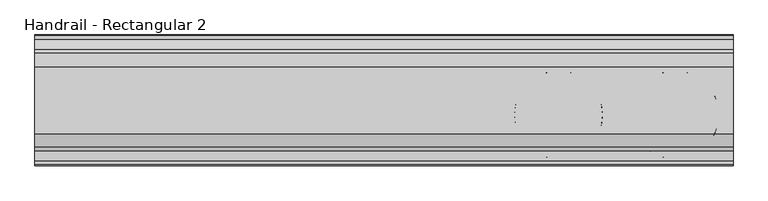
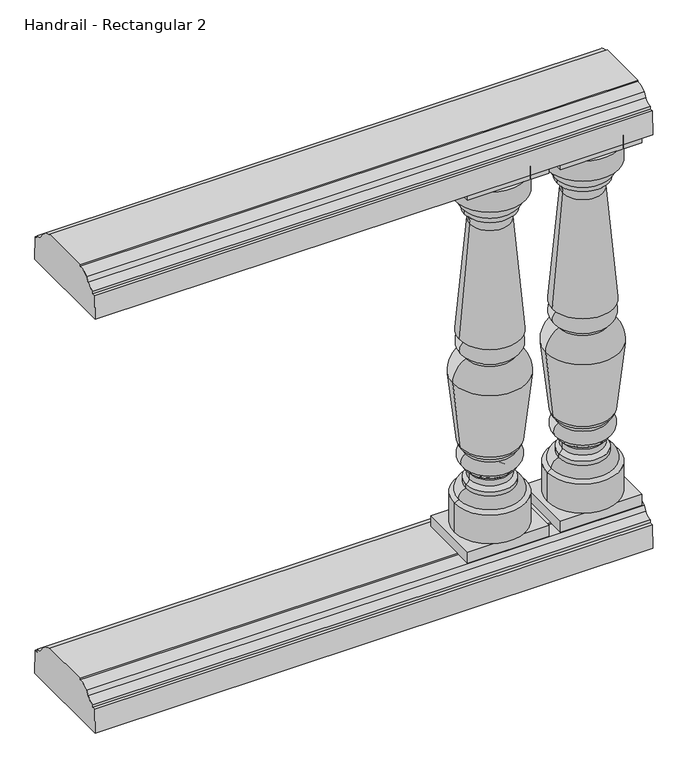
"""IFC4 building model written with IfcOpenShell, lengths in millimetres: railing geometry, Handrail - Rectangular 2."""

from ifc_helpers import new_model, si_unit, point, frame, frame_2d, origin, place, context, project, spatial, polyline, circle_curve, ellipse_curve, trimmed, segment, composite_curve, outline, extrude, source, transform, mapped, element, save
from ifc_brep_helpers import plane_surface, cylinder_surface, revolved_surface, advanced_brep


def handrail_rectangular_2_3b62de76(model_context):
    return source(origin(), model_context, "Body", "SolidModel", [
        extrude(outline(composite_curve([segment(trimmed(circle_curve(frame_2d((-1771.1852268, 1054.89375)), 19.84375), [point((-1771.1852268, 1035.05))], [point((-1754.064785, 1044.8605607))], True, "CARTESIAN"), True, "CONTINUOUS"), segment(polyline([(-1754.064785, 1044.8605607), (-1747.604713, 1054.3201059)]), True, "CONTINUOUS"), segment(trimmed(circle_curve(frame_2d((-1723.5602268, 1027.90625)), 35.71875), [point((-1747.604713, 1054.3201059))], [point((-1723.5602268, 1063.625))], False, "CARTESIAN"), True, "CONTINUOUS"), segment(polyline([(-1723.5602268, 1063.625), (-1723.5602268, 1066.8), (-1607.6727268, 1066.8), (-1607.6727268, 1063.625)]), True, "CONTINUOUS"), segment(trimmed(circle_curve(frame_2d((-1607.6727268, 1027.90625)), 35.71875), [point((-1607.6727268, 1063.625))], [point((-1583.6282406, 1054.3201059))], False, "CARTESIAN"), True, "CONTINUOUS"), segment(polyline([(-1583.6282406, 1054.3201059), (-1577.1681686, 1044.8605607)]), True, "CONTINUOUS"), segment(trimmed(circle_curve(frame_2d((-1560.0477268, 1054.89375)), 19.84375), [point((-1577.1681686, 1044.8605607))], [point((-1560.0477268, 1035.05))], True, "CARTESIAN"), True, "CONTINUOUS"), segment(polyline([(-1560.0477268, 1035.05), (-1560.0477268, 1028.7), (-1552.9039768, 1028.7), (-1551.3164768, 974.725), (-1779.9164768, 974.725), (-1778.3289768, 1028.7), (-1771.1852268, 1028.7), (-1771.1852268, 1035.05)]), True, "CONTINUOUS")], self_intersect=False)), frame((8950.8521895, 0.0, 0.0), z_axis=(1.0, 0.0, 0.0), x_axis=(0.0, 1.0, 0.0)), (0.0, 0.0, 1.0), 1219.2),
        extrude(outline(composite_curve([segment(trimmed(circle_curve(frame_2d((-1771.1852268, 99.21875)), 19.84375), [point((-1771.1852268, 79.375))], [point((-1754.064785, 89.1855607))], True, "CARTESIAN"), True, "CONTINUOUS"), segment(polyline([(-1754.064785, 89.1855607), (-1747.604713, 98.6451059)]), True, "CONTINUOUS"), segment(trimmed(circle_curve(frame_2d((-1723.5602268, 72.23125)), 35.71875), [point((-1747.604713, 98.6451059))], [point((-1723.5602268, 107.95))], False, "CARTESIAN"), True, "CONTINUOUS"), segment(polyline([(-1723.5602268, 107.95), (-1723.5602268, 111.125), (-1607.6727268, 111.125), (-1607.6727268, 107.95)]), True, "CONTINUOUS"), segment(trimmed(circle_curve(frame_2d((-1607.6727268, 72.23125)), 35.71875), [point((-1607.6727268, 107.95))], [point((-1583.6282406, 98.6451059))], False, "CARTESIAN"), True, "CONTINUOUS"), segment(polyline([(-1583.6282406, 98.6451059), (-1577.1681686, 89.1855607)]), True, "CONTINUOUS"), segment(trimmed(circle_curve(frame_2d((-1560.0477268, 99.21875)), 19.84375), [point((-1577.1681686, 89.1855607))], [point((-1560.0477268, 79.375))], True, "CARTESIAN"), True, "CONTINUOUS"), segment(polyline([(-1560.0477268, 79.375), (-1560.0477268, 73.025), (-1552.9039768, 73.025), (-1551.3164768, 19.05), (-1779.9164768, 19.05), (-1778.3289768, 73.025), (-1771.1852268, 73.025), (-1771.1852268, 79.375)]), True, "CONTINUOUS")], self_intersect=False)), frame((8950.8521895, 0.0, 0.0), z_axis=(1.0, 0.0, 0.0), x_axis=(0.0, 1.0, 0.0)), (0.0, 0.0, 1.0), 1219.2),
        advanced_brep(
        [(10068.4521895, -1691.0164768, 949.325), (9990.8909506, -1691.0164768, 949.325), (10146.0134284, -1691.0164768, 949.325), (10146.2396895, -1691.0164768, 136.525), (9990.6646895, -1691.0164768, 136.525), (10068.4521895, -1691.0164768, 136.525), (10146.2396895, -1691.0164768, 203.2), (9990.6646895, -1691.0164768, 203.2), (10136.6276556, -1691.0164768, 208.348485), (10000.2767235, -1691.0164768, 208.348485), (10120.8396895, -1691.0164768, 228.7310532), (10016.0646895, -1691.0164768, 228.7310532), (10120.8396895, -1691.0164768, 238.125), (10016.0646895, -1691.0164768, 238.125), (10113.2209727, -1691.0164768, 247.1598162), (10023.6834064, -1691.0164768, 247.1598162), (10113.2209727, -1691.0164768, 260.8401838), (10023.6834064, -1691.0164768, 260.8401838), (10120.8396895, -1691.0164768, 269.875), (10016.0646895, -1691.0164768, 269.875), (10120.8396895, -1691.0164768, 276.225), (10016.0646895, -1691.0164768, 276.225), (10121.6334395, -1691.0164768, 307.975), (10015.2709395, -1691.0164768, 307.975), (10121.6334395, -1691.0164768, 314.325), (10015.2709395, -1691.0164768, 314.325), (10132.4062243, -1691.0164768, 327.0157842), (10004.4981547, -1691.0164768, 327.0157842), (10149.493305, -1691.0164768, 481.3725887), (9987.4110741, -1691.0164768, 481.3725887), (10120.8396895, -1691.0164768, 528.6375), (10016.0646895, -1691.0164768, 528.6375), (10120.8396895, -1691.0164768, 534.9875), (10016.0646895, -1691.0164768, 534.9875), (10124.0146895, -1691.0164768, 569.9125), (10012.8896895, -1691.0164768, 569.9125), (10124.0146895, -1691.0164768, 573.0875), (10012.8896895, -1691.0164768, 573.0875), (10135.1271895, -1691.0164768, 577.85), (10001.7771895, -1691.0164768, 577.85), (10111.9486775, -1691.0164768, 836.3199218), (10024.9557016, -1691.0164768, 836.3199218), (10124.0146895, -1691.0164768, 863.6), (10012.8896895, -1691.0164768, 863.6), (10124.0146895, -1691.0164768, 873.125), (10012.8896895, -1691.0164768, 873.125), (10135.1271895, -1691.0164768, 900.1125), (10001.7771895, -1691.0164768, 900.1125), (10146.2396895, -1691.0164768, 903.2875), (9990.6646895, -1691.0164768, 903.2875)],
        [
            (0, 1),
            (1, 2, circle_curve(frame((10068.4521895, -1691.0164768, 949.325), z_axis=(0.0, 0.0, 1.0), x_axis=(-1.0, 0.0, 0.0)), 77.5612389)),
            (2, 0),
            (2, 1, circle_curve(frame((10068.4521895, -1691.0164768, 949.325), z_axis=(0.0, 0.0, 1.0), x_axis=(-1.0, 0.0, 0.0)), 77.5612389)),
            (3, 4, circle_curve(frame((10068.4521895, -1691.0164768, 136.525), z_axis=(0.0, 0.0, -1.0), x_axis=(-1.0, 0.0, 0.0)), 77.7875)),
            (4, 5),
            (5, 3),
            (4, 3, circle_curve(frame((10068.4521895, -1691.0164768, 136.525), z_axis=(0.0, 0.0, -1.0), x_axis=(-1.0, 0.0, 0.0)), 77.7875)),
            (6, 7, circle_curve(frame((10068.4521895, -1691.0164768, 203.2), z_axis=(0.0, 0.0, -1.0), x_axis=(-1.0, 0.0, 0.0)), 77.7875)),
            (7, 4),
            (3, 6),
            (7, 6, circle_curve(frame((10068.4521895, -1691.0164768, 203.2), z_axis=(0.0, 0.0, -1.0), x_axis=(-1.0, 0.0, 0.0)), 77.7875)),
            (8, 9, circle_curve(frame((10068.4521895, -1691.0164768, 208.348485), z_axis=(0.0, 0.0, -1.0), x_axis=(-1.0, 0.0, 0.0)), 68.175466)),
            (9, 7),
            (6, 8),
            (9, 8, circle_curve(frame((10068.4521895, -1691.0164768, 208.348485), z_axis=(0.0, 0.0, -1.0), x_axis=(-1.0, 0.0, 0.0)), 68.175466)),
            (10, 11, circle_curve(frame((10068.4521895, -1691.0164768, 228.7310532), z_axis=(0.0, 0.0, -1.0), x_axis=(-1.0, 0.0, 0.0)), 52.3875)),
            (11, 9, circle_curve(frame((10018.4397784, -1691.0164768, 210.5855331), z_axis=(0.0, -1.0, 0.0), x_axis=(1.0, 0.0, 0.0)), 18.3002991)),
            (8, 10, circle_curve(frame((10118.4646007, -1691.0164768, 210.5855331), z_axis=(0.0, -1.0, 0.0), x_axis=(-1.0, 0.0, 0.0)), 18.3002991)),
            (11, 10, circle_curve(frame((10068.4521895, -1691.0164768, 228.7310532), z_axis=(0.0, 0.0, -1.0), x_axis=(-1.0, 0.0, 0.0)), 52.3875)),
            (12, 13, circle_curve(frame((10068.4521895, -1691.0164768, 238.125), z_axis=(0.0, 0.0, -1.0), x_axis=(-1.0, 0.0, 0.0)), 52.3875)),
            (13, 11),
            (10, 12),
            (13, 12, circle_curve(frame((10068.4521895, -1691.0164768, 238.125), z_axis=(0.0, 0.0, -1.0), x_axis=(-1.0, 0.0, 0.0)), 52.3875)),
            (14, 15, circle_curve(frame((10068.4521895, -1691.0164768, 247.1598162), z_axis=(0.0, 0.0, -1.0), x_axis=(-1.0, 0.0, 0.0)), 44.7687831)),
            (15, 13, circle_curve(frame((10014.2793543, -1691.0164768, 247.3602005), z_axis=(0.0, 1.0, 0.0), x_axis=(1.0, 0.0, 0.0)), 9.4061868)),
            (12, 14, circle_curve(frame((10122.6250248, -1691.0164768, 247.3602005), z_axis=(0.0, 1.0, 0.0), x_axis=(-1.0, 0.0, 0.0)), 9.4061868)),
            (15, 14, circle_curve(frame((10068.4521895, -1691.0164768, 247.1598162), z_axis=(0.0, 0.0, -1.0), x_axis=(-1.0, 0.0, 0.0)), 44.7687831)),
            (16, 17, circle_curve(frame((10068.4521895, -1691.0164768, 260.8401838), z_axis=(0.0, 0.0, -1.0), x_axis=(-1.0, 0.0, 0.0)), 44.7687831)),
            (17, 15),
            (14, 16),
            (17, 16, circle_curve(frame((10068.4521895, -1691.0164768, 260.8401838), z_axis=(0.0, 0.0, -1.0), x_axis=(-1.0, 0.0, 0.0)), 44.7687831)),
            (18, 19, circle_curve(frame((10068.4521895, -1691.0164768, 269.875), z_axis=(0.0, 0.0, -1.0), x_axis=(-1.0, 0.0, 0.0)), 52.3875)),
            (19, 17, circle_curve(frame((10014.2793543, -1691.0164768, 260.6397995), z_axis=(0.0, 1.0, 0.0), x_axis=(1.0, 0.0, 0.0)), 9.4061868)),
            (16, 18, circle_curve(frame((10122.6250248, -1691.0164768, 260.6397995), z_axis=(0.0, 1.0, 0.0), x_axis=(-1.0, 0.0, 0.0)), 9.4061868)),
            (19, 18, circle_curve(frame((10068.4521895, -1691.0164768, 269.875), z_axis=(0.0, 0.0, -1.0), x_axis=(-1.0, 0.0, 0.0)), 52.3875)),
            (20, 21, circle_curve(frame((10068.4521895, -1691.0164768, 276.225), z_axis=(0.0, 0.0, -1.0), x_axis=(-1.0, 0.0, 0.0)), 52.3875)),
            (21, 19),
            (18, 20),
            (21, 20, circle_curve(frame((10068.4521895, -1691.0164768, 276.225), z_axis=(0.0, 0.0, -1.0), x_axis=(-1.0, 0.0, 0.0)), 52.3875)),
            (22, 23, circle_curve(frame((10068.4521895, -1691.0164768, 307.975), z_axis=(0.0, 0.0, -1.0), x_axis=(-1.0, 0.0, 0.0)), 53.18125)),
            (23, 21, circle_curve(frame((10021.6437772, -1691.0164768, 292.2493991), z_axis=(0.0, -1.0, 0.0), x_axis=(1.0, 0.0, 0.0)), 16.9678397)),
            (20, 22, circle_curve(frame((10115.2606019, -1691.0164768, 292.2493991), z_axis=(0.0, -1.0, 0.0), x_axis=(-1.0, 0.0, 0.0)), 16.9678397)),
            (23, 22, circle_curve(frame((10068.4521895, -1691.0164768, 307.975), z_axis=(0.0, 0.0, -1.0), x_axis=(-1.0, 0.0, 0.0)), 53.18125)),
            (24, 25, circle_curve(frame((10068.4521895, -1691.0164768, 314.325), z_axis=(0.0, 0.0, -1.0), x_axis=(-1.0, 0.0, 0.0)), 53.18125)),
            (25, 23),
            (22, 24),
            (25, 24, circle_curve(frame((10068.4521895, -1691.0164768, 314.325), z_axis=(0.0, 0.0, -1.0), x_axis=(-1.0, 0.0, 0.0)), 53.18125)),
            (26, 27, circle_curve(frame((10068.4521895, -1691.0164768, 327.0157842), z_axis=(0.0, 0.0, -1.0), x_axis=(-1.0, 0.0, 0.0)), 63.9540348)),
            (27, 25, circle_curve(frame((10025.104312, -1691.0164768, 333.5899445), z_axis=(0.0, -1.0, 0.0), x_axis=(1.0, 0.0, 0.0)), 21.6294545)),
            (24, 26, circle_curve(frame((10111.8000671, -1691.0164768, 333.5899445), z_axis=(0.0, -1.0, 0.0), x_axis=(-1.0, 0.0, 0.0)), 21.6294545)),
            (27, 26, circle_curve(frame((10068.4521895, -1691.0164768, 327.0157842), z_axis=(0.0, 0.0, -1.0), x_axis=(-1.0, 0.0, 0.0)), 63.9540348)),
            (28, 29, circle_curve(frame((10068.4521895, -1691.0164768, 481.3725887), z_axis=(0.0, 0.0, -1.0), x_axis=(-1.0, 0.0, 0.0)), 81.0411154)),
            (29, 27, circle_curve(frame((11481.7385198, -1691.0164768, 568.6683698), z_axis=(0.0, -1.0, 0.0), x_axis=(1.0, 0.0, 0.0)), 1496.8751012)),
            (26, 28, circle_curve(frame((8655.1658592, -1691.0164768, 568.6683698), z_axis=(0.0, -1.0, 0.0), x_axis=(-1.0, 0.0, 0.0)), 1496.8751012)),
            (29, 28, circle_curve(frame((10068.4521895, -1691.0164768, 481.3725887), z_axis=(0.0, 0.0, -1.0), x_axis=(-1.0, 0.0, 0.0)), 81.0411154)),
            (30, 31, circle_curve(frame((10068.4521895, -1691.0164768, 528.6375), z_axis=(0.0, 0.0, -1.0), x_axis=(-1.0, 0.0, 0.0)), 52.3875)),
            (31, 29, circle_curve(frame((10039.1638402, -1691.0164768, 482.3161407), z_axis=(0.0, -1.0, 0.0), x_axis=(1.0, 0.0, 0.0)), 51.7613668)),
            (28, 30, circle_curve(frame((10097.7405389, -1691.0164768, 482.3161407), z_axis=(0.0, -1.0, 0.0), x_axis=(-1.0, 0.0, 0.0)), 51.7613668)),
            (31, 30, circle_curve(frame((10068.4521895, -1691.0164768, 528.6375), z_axis=(0.0, 0.0, -1.0), x_axis=(-1.0, 0.0, 0.0)), 52.3875)),
            (32, 33, circle_curve(frame((10068.4521895, -1691.0164768, 534.9875), z_axis=(0.0, 0.0, -1.0), x_axis=(-1.0, 0.0, 0.0)), 52.3875)),
            (33, 31),
            (30, 32),
            (33, 32, circle_curve(frame((10068.4521895, -1691.0164768, 534.9875), z_axis=(0.0, 0.0, -1.0), x_axis=(-1.0, 0.0, 0.0)), 52.3875)),
            (34, 35, circle_curve(frame((10068.4521895, -1691.0164768, 569.9125), z_axis=(0.0, 0.0, -1.0), x_axis=(-1.0, 0.0, 0.0)), 55.5625)),
            (35, 33, circle_curve(frame((10021.1309419, -1691.0164768, 553.0548866), z_axis=(0.0, -1.0, 0.0), x_axis=(1.0, 0.0, 0.0)), 18.7642578)),
            (32, 34, circle_curve(frame((10115.7734372, -1691.0164768, 553.0548866), z_axis=(0.0, -1.0, 0.0), x_axis=(-1.0, 0.0, 0.0)), 18.7642578)),
            (35, 34, circle_curve(frame((10068.4521895, -1691.0164768, 569.9125), z_axis=(0.0, 0.0, -1.0), x_axis=(-1.0, 0.0, 0.0)), 55.5625)),
            (36, 37, circle_curve(frame((10068.4521895, -1691.0164768, 573.0875), z_axis=(0.0, 0.0, -1.0), x_axis=(-1.0, 0.0, 0.0)), 55.5625)),
            (37, 35),
            (34, 36),
            (37, 36, circle_curve(frame((10068.4521895, -1691.0164768, 573.0875), z_axis=(0.0, 0.0, -1.0), x_axis=(-1.0, 0.0, 0.0)), 55.5625)),
            (38, 39, circle_curve(frame((10068.4521895, -1691.0164768, 577.85), z_axis=(0.0, 0.0, -1.0), x_axis=(-1.0, 0.0, 0.0)), 66.675)),
            (39, 37),
            (36, 38),
            (39, 38, circle_curve(frame((10068.4521895, -1691.0164768, 577.85), z_axis=(0.0, 0.0, -1.0), x_axis=(-1.0, 0.0, 0.0)), 66.675)),
            (40, 41, circle_curve(frame((10068.4521895, -1691.0164768, 836.3199218), z_axis=(0.0, 0.0, -1.0), x_axis=(-1.0, 0.0, 0.0)), 43.4964879)),
            (41, 39, circle_curve(frame((8378.1192757, -1691.0164768, 853.7271544), z_axis=(0.0, 1.0, 0.0), x_axis=(1.0, 0.0, 0.0)), 1646.9284215)),
            (38, 40, circle_curve(frame((11758.7851034, -1691.0164768, 853.7271544), z_axis=(0.0, 1.0, 0.0), x_axis=(-1.0, 0.0, 0.0)), 1646.9284215)),
            (41, 40, circle_curve(frame((10068.4521895, -1691.0164768, 836.3199218), z_axis=(0.0, 0.0, -1.0), x_axis=(-1.0, 0.0, 0.0)), 43.4964879)),
            (42, 43, circle_curve(frame((10068.4521895, -1691.0164768, 863.6), z_axis=(0.0, 0.0, -1.0), x_axis=(-1.0, 0.0, 0.0)), 55.5625)),
            (43, 41, circle_curve(frame((9992.2515427, -1691.0164768, 838.1632773), z_axis=(0.0, 1.0, 0.0), x_axis=(1.0, 0.0, 0.0)), 32.7560676)),
            (40, 42, circle_curve(frame((10144.6528363, -1691.0164768, 838.1632773), z_axis=(0.0, 1.0, 0.0), x_axis=(-1.0, 0.0, 0.0)), 32.7560676)),
            (43, 42, circle_curve(frame((10068.4521895, -1691.0164768, 863.6), z_axis=(0.0, 0.0, -1.0), x_axis=(-1.0, 0.0, 0.0)), 55.5625)),
            (44, 45, circle_curve(frame((10068.4521895, -1691.0164768, 873.125), z_axis=(0.0, 0.0, -1.0), x_axis=(-1.0, 0.0, 0.0)), 55.5625)),
            (45, 43),
            (42, 44),
            (45, 44, circle_curve(frame((10068.4521895, -1691.0164768, 873.125), z_axis=(0.0, 0.0, -1.0), x_axis=(-1.0, 0.0, 0.0)), 55.5625)),
            (46, 47, circle_curve(frame((10068.4521895, -1691.0164768, 900.1125), z_axis=(0.0, 0.0, -1.0), x_axis=(-1.0, 0.0, 0.0)), 66.675)),
            (47, 45, circle_curve(frame((10031.1374113, -1691.0164768, 896.4203854), z_axis=(0.0, -1.0, 0.0), x_axis=(1.0, 0.0, 0.0)), 29.5914571)),
            (44, 46, circle_curve(frame((10105.7669678, -1691.0164768, 896.4203854), z_axis=(0.0, -1.0, 0.0), x_axis=(-1.0, 0.0, 0.0)), 29.5914571)),
            (47, 46, circle_curve(frame((10068.4521895, -1691.0164768, 900.1125), z_axis=(0.0, 0.0, -1.0), x_axis=(-1.0, 0.0, 0.0)), 66.675)),
            (48, 49, circle_curve(frame((10068.4521895, -1691.0164768, 903.2875), z_axis=(0.0, 0.0, -1.0), x_axis=(-1.0, 0.0, 0.0)), 77.7875)),
            (49, 47),
            (46, 48),
            (49, 48, circle_curve(frame((10068.4521895, -1691.0164768, 903.2875), z_axis=(0.0, 0.0, -1.0), x_axis=(-1.0, 0.0, 0.0)), 77.7875)),
            (1, 49),
            (48, 2),
        ],
        [
            plane_surface(frame((10068.4521895, -1691.0164768, 949.325), z_axis=(0.0, 0.0, 1.0), x_axis=(-1.0, 0.0, 0.0))),
            plane_surface(frame((10068.4521895, -1691.0164768, 136.525), z_axis=(0.0, 0.0, -1.0), x_axis=(-1.0, 0.0, 0.0))),
            cylinder_surface(frame((10068.4521895, -1691.0164768, 1019.175), z_axis=(0.0, 0.0, 1.0), x_axis=(-1.0, 0.0, 0.0)), 77.7875),
            revolved_surface(polyline([(9990.6646895, -1691.0164768, 203.2), (10000.2767235, -1691.0164768, 208.348485)]), (10068.4521895, -1691.0164768, 1019.175), (0.0, 0.0, 1.0)),
            revolved_surface(trimmed(ellipse_curve(frame((10018.4397784, -1691.0164768, 210.5855331), z_axis=(0.0, 1.0, 0.0), x_axis=(1.0, 0.0, 0.0)), 18.3002991, 18.3002991), [point((10000.2767235, -1691.0164768, 208.348485))], [point((10016.0646895, -1691.0164768, 228.7310532))], True, "CARTESIAN"), (10068.4521895, -1691.0164768, 1019.175), (0.0, 0.0, 1.0)),
            cylinder_surface(frame((10068.4521895, -1691.0164768, 1019.175), z_axis=(0.0, 0.0, 1.0), x_axis=(-1.0, 0.0, 0.0)), 52.3875),
            revolved_surface(trimmed(ellipse_curve(frame((10014.2793543, -1691.0164768, 247.3602005), z_axis=(0.0, -1.0, 0.0), x_axis=(1.0, 0.0, 0.0)), 9.4061868, 9.4061868), [point((10016.0646895, -1691.0164768, 238.125))], [point((10023.6834064, -1691.0164768, 247.1598162))], True, "CARTESIAN"), (10068.4521895, -1691.0164768, 1019.175), (0.0, 0.0, 1.0)),
            cylinder_surface(frame((10068.4521895, -1691.0164768, 1019.175), z_axis=(0.0, 0.0, 1.0), x_axis=(-1.0, 0.0, 0.0)), 44.7687831),
            revolved_surface(trimmed(ellipse_curve(frame((10014.2793543, -1691.0164768, 260.6397995), z_axis=(0.0, -1.0, 0.0), x_axis=(1.0, 0.0, 0.0)), 9.4061868, 9.4061868), [point((10023.6834064, -1691.0164768, 260.8401838))], [point((10016.0646895, -1691.0164768, 269.875))], True, "CARTESIAN"), (10068.4521895, -1691.0164768, 1019.175), (0.0, 0.0, 1.0)),
            revolved_surface(trimmed(ellipse_curve(frame((10021.6437772, -1691.0164768, 292.2493991), z_axis=(0.0, 1.0, 0.0), x_axis=(1.0, 0.0, 0.0)), 16.9678397, 16.9678397), [point((10016.0646895, -1691.0164768, 276.225))], [point((10015.2709395, -1691.0164768, 307.975))], True, "CARTESIAN"), (10068.4521895, -1691.0164768, 1019.175), (0.0, 0.0, 1.0)),
            cylinder_surface(frame((10068.4521895, -1691.0164768, 1019.175), z_axis=(0.0, 0.0, 1.0), x_axis=(-1.0, 0.0, 0.0)), 53.18125),
            revolved_surface(trimmed(ellipse_curve(frame((10025.104312, -1691.0164768, 333.5899445), z_axis=(0.0, 1.0, 0.0), x_axis=(1.0, 0.0, 0.0)), 21.6294545, 21.6294545), [point((10015.2709395, -1691.0164768, 314.325))], [point((10004.4981547, -1691.0164768, 327.0157842))], True, "CARTESIAN"), (10068.4521895, -1691.0164768, 1019.175), (0.0, 0.0, 1.0)),
            revolved_surface(trimmed(ellipse_curve(frame((11481.7385198, -1691.0164768, 568.6683698), z_axis=(0.0, 1.0, 0.0), x_axis=(1.0, 0.0, 0.0)), 1496.8751012, 1496.8751012), [point((10004.4981547, -1691.0164768, 327.0157842))], [point((9987.4110741, -1691.0164768, 481.3725887))], True, "CARTESIAN"), (10068.4521895, -1691.0164768, 1019.175), (0.0, 0.0, 1.0)),
            revolved_surface(trimmed(ellipse_curve(frame((10039.1638402, -1691.0164768, 482.3161407), z_axis=(0.0, 1.0, 0.0), x_axis=(1.0, 0.0, 0.0)), 51.7613668, 51.7613668), [point((9987.4110741, -1691.0164768, 481.3725887))], [point((10016.0646895, -1691.0164768, 528.6375))], True, "CARTESIAN"), (10068.4521895, -1691.0164768, 1019.175), (0.0, 0.0, 1.0)),
            revolved_surface(trimmed(ellipse_curve(frame((10021.1309419, -1691.0164768, 553.0548866), z_axis=(0.0, 1.0, 0.0), x_axis=(1.0, 0.0, 0.0)), 18.7642578, 18.7642578), [point((10016.0646895, -1691.0164768, 534.9875))], [point((10012.8896895, -1691.0164768, 569.9125))], True, "CARTESIAN"), (10068.4521895, -1691.0164768, 1019.175), (0.0, 0.0, 1.0)),
            cylinder_surface(frame((10068.4521895, -1691.0164768, 1019.175), z_axis=(0.0, 0.0, 1.0), x_axis=(-1.0, 0.0, 0.0)), 55.5625),
            revolved_surface(polyline([(10012.8896895, -1691.0164768, 573.0875), (10001.7771895, -1691.0164768, 577.85)]), (10068.4521895, -1691.0164768, 1019.175), (0.0, 0.0, 1.0)),
            revolved_surface(trimmed(ellipse_curve(frame((8378.1192757, -1691.0164768, 853.7271544), z_axis=(0.0, -1.0, 0.0), x_axis=(1.0, 0.0, 0.0)), 1646.9284215, 1646.9284215), [point((10001.7771895, -1691.0164768, 577.85))], [point((10024.9557016, -1691.0164768, 836.3199218))], True, "CARTESIAN"), (10068.4521895, -1691.0164768, 1019.175), (0.0, 0.0, 1.0)),
            revolved_surface(trimmed(ellipse_curve(frame((9992.2515427, -1691.0164768, 838.1632773), z_axis=(0.0, -1.0, 0.0), x_axis=(1.0, 0.0, 0.0)), 32.7560676, 32.7560676), [point((10024.9557016, -1691.0164768, 836.3199218))], [point((10012.8896895, -1691.0164768, 863.6))], True, "CARTESIAN"), (10068.4521895, -1691.0164768, 1019.175), (0.0, 0.0, 1.0)),
            revolved_surface(trimmed(ellipse_curve(frame((10031.1374113, -1691.0164768, 896.4203854), z_axis=(0.0, 1.0, 0.0), x_axis=(1.0, 0.0, 0.0)), 29.5914571, 29.5914571), [point((10012.8896895, -1691.0164768, 873.125))], [point((10001.7771895, -1691.0164768, 900.1125))], True, "CARTESIAN"), (10068.4521895, -1691.0164768, 1019.175), (0.0, 0.0, 1.0)),
            revolved_surface(polyline([(10001.7771895, -1691.0164768, 900.1125), (9990.6646895, -1691.0164768, 903.2875)]), (10068.4521895, -1691.0164768, 1019.175), (0.0, 0.0, 1.0)),
            revolved_surface(polyline([(9990.6646895, -1691.0164768, 903.2875), (9990.8909506, -1691.0164768, 949.325)]), (10068.4521895, -1691.0164768, 1019.175), (0.0, 0.0, 1.0)),
        ],
        [
            (0, [[1, 2, 3]]),
            (0, [[-3, 4, -1]]),
            (1, [[5, 6, 7]]),
            (1, [[8, -7, -6]]),
            (2, [[9, 10, -5, 11]]),
            (2, [[12, -11, -8, -10]]),
            (3, [[13, 14, -9, 15]]),
            (3, [[16, -15, -12, -14]]),
            (4, [[17, 18, -13, 19]]),
            (4, [[20, -19, -16, -18]]),
            (5, [[21, 22, -17, 23]]),
            (5, [[24, -23, -20, -22]]),
            (6, [[25, 26, -21, 27]]),
            (6, [[28, -27, -24, -26]]),
            (7, [[29, 30, -25, 31]]),
            (7, [[32, -31, -28, -30]]),
            (8, [[33, 34, -29, 35]]),
            (8, [[36, -35, -32, -34]]),
            (5, [[37, 38, -33, 39]]),
            (5, [[40, -39, -36, -38]]),
            (9, [[41, 42, -37, 43]]),
            (9, [[44, -43, -40, -42]]),
            (10, [[45, 46, -41, 47]]),
            (10, [[48, -47, -44, -46]]),
            (11, [[49, 50, -45, 51]]),
            (11, [[52, -51, -48, -50]]),
            (12, [[53, 54, -49, 55]]),
            (12, [[56, -55, -52, -54]]),
            (13, [[57, 58, -53, 59]]),
            (13, [[60, -59, -56, -58]]),
            (5, [[61, 62, -57, 63]]),
            (5, [[64, -63, -60, -62]]),
            (14, [[65, 66, -61, 67]]),
            (14, [[68, -67, -64, -66]]),
            (15, [[69, 70, -65, 71]]),
            (15, [[72, -71, -68, -70]]),
            (16, [[73, 74, -69, 75]]),
            (16, [[76, -75, -72, -74]]),
            (17, [[77, 78, -73, 79]]),
            (17, [[80, -79, -76, -78]]),
            (18, [[81, 82, -77, 83]]),
            (18, [[84, -83, -80, -82]]),
            (15, [[85, 86, -81, 87]]),
            (15, [[88, -87, -84, -86]]),
            (19, [[89, 90, -85, 91]]),
            (19, [[92, -91, -88, -90]]),
            (20, [[93, 94, -89, 95]]),
            (20, [[96, -95, -92, -94]]),
            (21, [[-2, 97, -93, 98]]),
            (21, [[-4, -98, -96, -97]]),
        ],
    ),
        extrude(outline(polyline([(9979.5521895, -1760.8664768), (9979.5521895, -1621.1664768), (10157.3521895, -1621.1664768), (10157.3521895, -1760.8664768), (9979.5521895, -1760.8664768)])), frame((0.0, 0.0, 111.125), z_axis=(0.0, 0.0, 1.0), x_axis=(1.0, 0.0, 0.0)), (0.0, 0.0, 1.0), 25.4),
        extrude(outline(polyline([(9979.5521895, -1621.1664768), (10157.3521895, -1621.1664768), (10157.3521895, -1760.8664768), (9979.5521895, -1760.8664768), (9979.5521895, -1621.1664768)])), frame((0.0, 0.0, 949.325), z_axis=(0.0, 0.0, 1.0), x_axis=(1.0, 0.0, 0.0)), (0.0, 0.0, 1.0), 25.4),
        advanced_brep(
        [(9865.2521895, -1691.0164768, 949.325), (9787.6909506, -1691.0164768, 949.325), (9942.8134284, -1691.0164768, 949.325), (9943.0396895, -1691.0164768, 136.525), (9787.4646895, -1691.0164768, 136.525), (9865.2521895, -1691.0164768, 136.525), (9943.0396895, -1691.0164768, 203.2), (9787.4646895, -1691.0164768, 203.2), (9933.4276556, -1691.0164768, 208.348485), (9797.0767235, -1691.0164768, 208.348485), (9917.6396895, -1691.0164768, 228.7310532), (9812.8646895, -1691.0164768, 228.7310532), (9917.6396895, -1691.0164768, 238.125), (9812.8646895, -1691.0164768, 238.125), (9910.0209727, -1691.0164768, 247.1598162), (9820.4834064, -1691.0164768, 247.1598162), (9910.0209727, -1691.0164768, 260.8401838), (9820.4834064, -1691.0164768, 260.8401838), (9917.6396895, -1691.0164768, 269.875), (9812.8646895, -1691.0164768, 269.875), (9917.6396895, -1691.0164768, 276.225), (9812.8646895, -1691.0164768, 276.225), (9918.4334395, -1691.0164768, 307.975), (9812.0709395, -1691.0164768, 307.975), (9918.4334395, -1691.0164768, 314.325), (9812.0709395, -1691.0164768, 314.325), (9929.2062243, -1691.0164768, 327.0157842), (9801.2981547, -1691.0164768, 327.0157842), (9946.293305, -1691.0164768, 481.3725887), (9784.2110741, -1691.0164768, 481.3725887), (9917.6396895, -1691.0164768, 528.6375), (9812.8646895, -1691.0164768, 528.6375), (9917.6396895, -1691.0164768, 534.9875), (9812.8646895, -1691.0164768, 534.9875), (9920.8146895, -1691.0164768, 569.9125), (9809.6896895, -1691.0164768, 569.9125), (9920.8146895, -1691.0164768, 573.0875), (9809.6896895, -1691.0164768, 573.0875), (9931.9271895, -1691.0164768, 577.85), (9798.5771895, -1691.0164768, 577.85), (9908.7486775, -1691.0164768, 836.3199218), (9821.7557016, -1691.0164768, 836.3199218), (9920.8146895, -1691.0164768, 863.6), (9809.6896895, -1691.0164768, 863.6), (9920.8146895, -1691.0164768, 873.125), (9809.6896895, -1691.0164768, 873.125), (9931.9271895, -1691.0164768, 900.1125), (9798.5771895, -1691.0164768, 900.1125), (9943.0396895, -1691.0164768, 903.2875), (9787.4646895, -1691.0164768, 903.2875)],
        [
            (0, 1),
            (1, 2, circle_curve(frame((9865.2521895, -1691.0164768, 949.325), z_axis=(0.0, 0.0, 1.0), x_axis=(-1.0, 0.0, 0.0)), 77.5612389)),
            (2, 0),
            (2, 1, circle_curve(frame((9865.2521895, -1691.0164768, 949.325), z_axis=(0.0, 0.0, 1.0), x_axis=(-1.0, 0.0, 0.0)), 77.5612389)),
            (3, 4, circle_curve(frame((9865.2521895, -1691.0164768, 136.525), z_axis=(0.0, 0.0, -1.0), x_axis=(-1.0, 0.0, 0.0)), 77.7875)),
            (4, 5),
            (5, 3),
            (4, 3, circle_curve(frame((9865.2521895, -1691.0164768, 136.525), z_axis=(0.0, 0.0, -1.0), x_axis=(-1.0, 0.0, 0.0)), 77.7875)),
            (6, 7, circle_curve(frame((9865.2521895, -1691.0164768, 203.2), z_axis=(0.0, 0.0, -1.0), x_axis=(-1.0, 0.0, 0.0)), 77.7875)),
            (7, 4),
            (3, 6),
            (7, 6, circle_curve(frame((9865.2521895, -1691.0164768, 203.2), z_axis=(0.0, 0.0, -1.0), x_axis=(-1.0, 0.0, 0.0)), 77.7875)),
            (8, 9, circle_curve(frame((9865.2521895, -1691.0164768, 208.348485), z_axis=(0.0, 0.0, -1.0), x_axis=(-1.0, 0.0, 0.0)), 68.175466)),
            (9, 7),
            (6, 8),
            (9, 8, circle_curve(frame((9865.2521895, -1691.0164768, 208.348485), z_axis=(0.0, 0.0, -1.0), x_axis=(-1.0, 0.0, 0.0)), 68.175466)),
            (10, 11, circle_curve(frame((9865.2521895, -1691.0164768, 228.7310532), z_axis=(0.0, 0.0, -1.0), x_axis=(-1.0, 0.0, 0.0)), 52.3875)),
            (11, 9, circle_curve(frame((9815.2397784, -1691.0164768, 210.5855331), z_axis=(0.0, -1.0, 0.0), x_axis=(1.0, 0.0, 0.0)), 18.3002991)),
            (8, 10, circle_curve(frame((9915.2646007, -1691.0164768, 210.5855331), z_axis=(0.0, -1.0, 0.0), x_axis=(-1.0, 0.0, 0.0)), 18.3002991)),
            (11, 10, circle_curve(frame((9865.2521895, -1691.0164768, 228.7310532), z_axis=(0.0, 0.0, -1.0), x_axis=(-1.0, 0.0, 0.0)), 52.3875)),
            (12, 13, circle_curve(frame((9865.2521895, -1691.0164768, 238.125), z_axis=(0.0, 0.0, -1.0), x_axis=(-1.0, 0.0, 0.0)), 52.3875)),
            (13, 11),
            (10, 12),
            (13, 12, circle_curve(frame((9865.2521895, -1691.0164768, 238.125), z_axis=(0.0, 0.0, -1.0), x_axis=(-1.0, 0.0, 0.0)), 52.3875)),
            (14, 15, circle_curve(frame((9865.2521895, -1691.0164768, 247.1598162), z_axis=(0.0, 0.0, -1.0), x_axis=(-1.0, 0.0, 0.0)), 44.7687831)),
            (15, 13, circle_curve(frame((9811.0793543, -1691.0164768, 247.3602005), z_axis=(0.0, 1.0, 0.0), x_axis=(1.0, 0.0, 0.0)), 9.4061868)),
            (12, 14, circle_curve(frame((9919.4250248, -1691.0164768, 247.3602005), z_axis=(0.0, 1.0, 0.0), x_axis=(-1.0, 0.0, 0.0)), 9.4061868)),
            (15, 14, circle_curve(frame((9865.2521895, -1691.0164768, 247.1598162), z_axis=(0.0, 0.0, -1.0), x_axis=(-1.0, 0.0, 0.0)), 44.7687831)),
            (16, 17, circle_curve(frame((9865.2521895, -1691.0164768, 260.8401838), z_axis=(0.0, 0.0, -1.0), x_axis=(-1.0, 0.0, 0.0)), 44.7687831)),
            (17, 15),
            (14, 16),
            (17, 16, circle_curve(frame((9865.2521895, -1691.0164768, 260.8401838), z_axis=(0.0, 0.0, -1.0), x_axis=(-1.0, 0.0, 0.0)), 44.7687831)),
            (18, 19, circle_curve(frame((9865.2521895, -1691.0164768, 269.875), z_axis=(0.0, 0.0, -1.0), x_axis=(-1.0, 0.0, 0.0)), 52.3875)),
            (19, 17, circle_curve(frame((9811.0793543, -1691.0164768, 260.6397995), z_axis=(0.0, 1.0, 0.0), x_axis=(1.0, 0.0, 0.0)), 9.4061868)),
            (16, 18, circle_curve(frame((9919.4250248, -1691.0164768, 260.6397995), z_axis=(0.0, 1.0, 0.0), x_axis=(-1.0, 0.0, 0.0)), 9.4061868)),
            (19, 18, circle_curve(frame((9865.2521895, -1691.0164768, 269.875), z_axis=(0.0, 0.0, -1.0), x_axis=(-1.0, 0.0, 0.0)), 52.3875)),
            (20, 21, circle_curve(frame((9865.2521895, -1691.0164768, 276.225), z_axis=(0.0, 0.0, -1.0), x_axis=(-1.0, 0.0, 0.0)), 52.3875)),
            (21, 19),
            (18, 20),
            (21, 20, circle_curve(frame((9865.2521895, -1691.0164768, 276.225), z_axis=(0.0, 0.0, -1.0), x_axis=(-1.0, 0.0, 0.0)), 52.3875)),
            (22, 23, circle_curve(frame((9865.2521895, -1691.0164768, 307.975), z_axis=(0.0, 0.0, -1.0), x_axis=(-1.0, 0.0, 0.0)), 53.18125)),
            (23, 21, circle_curve(frame((9818.4437772, -1691.0164768, 292.2493991), z_axis=(0.0, -1.0, 0.0), x_axis=(1.0, 0.0, 0.0)), 16.9678397)),
            (20, 22, circle_curve(frame((9912.0606019, -1691.0164768, 292.2493991), z_axis=(0.0, -1.0, 0.0), x_axis=(-1.0, 0.0, 0.0)), 16.9678397)),
            (23, 22, circle_curve(frame((9865.2521895, -1691.0164768, 307.975), z_axis=(0.0, 0.0, -1.0), x_axis=(-1.0, 0.0, 0.0)), 53.18125)),
            (24, 25, circle_curve(frame((9865.2521895, -1691.0164768, 314.325), z_axis=(0.0, 0.0, -1.0), x_axis=(-1.0, 0.0, 0.0)), 53.18125)),
            (25, 23),
            (22, 24),
            (25, 24, circle_curve(frame((9865.2521895, -1691.0164768, 314.325), z_axis=(0.0, 0.0, -1.0), x_axis=(-1.0, 0.0, 0.0)), 53.18125)),
            (26, 27, circle_curve(frame((9865.2521895, -1691.0164768, 327.0157842), z_axis=(0.0, 0.0, -1.0), x_axis=(-1.0, 0.0, 0.0)), 63.9540348)),
            (27, 25, circle_curve(frame((9821.904312, -1691.0164768, 333.5899445), z_axis=(0.0, -1.0, 0.0), x_axis=(1.0, 0.0, 0.0)), 21.6294545)),
            (24, 26, circle_curve(frame((9908.6000671, -1691.0164768, 333.5899445), z_axis=(0.0, -1.0, 0.0), x_axis=(-1.0, 0.0, 0.0)), 21.6294545)),
            (27, 26, circle_curve(frame((9865.2521895, -1691.0164768, 327.0157842), z_axis=(0.0, 0.0, -1.0), x_axis=(-1.0, 0.0, 0.0)), 63.9540348)),
            (28, 29, circle_curve(frame((9865.2521895, -1691.0164768, 481.3725887), z_axis=(0.0, 0.0, -1.0), x_axis=(-1.0, 0.0, 0.0)), 81.0411154)),
            (29, 27, circle_curve(frame((11278.5385198, -1691.0164768, 568.6683698), z_axis=(0.0, -1.0, 0.0), x_axis=(1.0, 0.0, 0.0)), 1496.8751012)),
            (26, 28, circle_curve(frame((8451.9658592, -1691.0164768, 568.6683698), z_axis=(0.0, -1.0, 0.0), x_axis=(-1.0, 0.0, 0.0)), 1496.8751012)),
            (29, 28, circle_curve(frame((9865.2521895, -1691.0164768, 481.3725887), z_axis=(0.0, 0.0, -1.0), x_axis=(-1.0, 0.0, 0.0)), 81.0411154)),
            (30, 31, circle_curve(frame((9865.2521895, -1691.0164768, 528.6375), z_axis=(0.0, 0.0, -1.0), x_axis=(-1.0, 0.0, 0.0)), 52.3875)),
            (31, 29, circle_curve(frame((9835.9638402, -1691.0164768, 482.3161407), z_axis=(0.0, -1.0, 0.0), x_axis=(1.0, 0.0, 0.0)), 51.7613668)),
            (28, 30, circle_curve(frame((9894.5405389, -1691.0164768, 482.3161407), z_axis=(0.0, -1.0, 0.0), x_axis=(-1.0, 0.0, 0.0)), 51.7613668)),
            (31, 30, circle_curve(frame((9865.2521895, -1691.0164768, 528.6375), z_axis=(0.0, 0.0, -1.0), x_axis=(-1.0, 0.0, 0.0)), 52.3875)),
            (32, 33, circle_curve(frame((9865.2521895, -1691.0164768, 534.9875), z_axis=(0.0, 0.0, -1.0), x_axis=(-1.0, 0.0, 0.0)), 52.3875)),
            (33, 31),
            (30, 32),
            (33, 32, circle_curve(frame((9865.2521895, -1691.0164768, 534.9875), z_axis=(0.0, 0.0, -1.0), x_axis=(-1.0, 0.0, 0.0)), 52.3875)),
            (34, 35, circle_curve(frame((9865.2521895, -1691.0164768, 569.9125), z_axis=(0.0, 0.0, -1.0), x_axis=(-1.0, 0.0, 0.0)), 55.5625)),
            (35, 33, circle_curve(frame((9817.9309419, -1691.0164768, 553.0548866), z_axis=(0.0, -1.0, 0.0), x_axis=(1.0, 0.0, 0.0)), 18.7642578)),
            (32, 34, circle_curve(frame((9912.5734372, -1691.0164768, 553.0548866), z_axis=(0.0, -1.0, 0.0), x_axis=(-1.0, 0.0, 0.0)), 18.7642578)),
            (35, 34, circle_curve(frame((9865.2521895, -1691.0164768, 569.9125), z_axis=(0.0, 0.0, -1.0), x_axis=(-1.0, 0.0, 0.0)), 55.5625)),
            (36, 37, circle_curve(frame((9865.2521895, -1691.0164768, 573.0875), z_axis=(0.0, 0.0, -1.0), x_axis=(-1.0, 0.0, 0.0)), 55.5625)),
            (37, 35),
            (34, 36),
            (37, 36, circle_curve(frame((9865.2521895, -1691.0164768, 573.0875), z_axis=(0.0, 0.0, -1.0), x_axis=(-1.0, 0.0, 0.0)), 55.5625)),
            (38, 39, circle_curve(frame((9865.2521895, -1691.0164768, 577.85), z_axis=(0.0, 0.0, -1.0), x_axis=(-1.0, 0.0, 0.0)), 66.675)),
            (39, 37),
            (36, 38),
            (39, 38, circle_curve(frame((9865.2521895, -1691.0164768, 577.85), z_axis=(0.0, 0.0, -1.0), x_axis=(-1.0, 0.0, 0.0)), 66.675)),
            (40, 41, circle_curve(frame((9865.2521895, -1691.0164768, 836.3199218), z_axis=(0.0, 0.0, -1.0), x_axis=(-1.0, 0.0, 0.0)), 43.4964879)),
            (41, 39, circle_curve(frame((8174.9192757, -1691.0164768, 853.7271544), z_axis=(0.0, 1.0, 0.0), x_axis=(1.0, 0.0, 0.0)), 1646.9284215)),
            (38, 40, circle_curve(frame((11555.5851034, -1691.0164768, 853.7271544), z_axis=(0.0, 1.0, 0.0), x_axis=(-1.0, 0.0, 0.0)), 1646.9284215)),
            (41, 40, circle_curve(frame((9865.2521895, -1691.0164768, 836.3199218), z_axis=(0.0, 0.0, -1.0), x_axis=(-1.0, 0.0, 0.0)), 43.4964879)),
            (42, 43, circle_curve(frame((9865.2521895, -1691.0164768, 863.6), z_axis=(0.0, 0.0, -1.0), x_axis=(-1.0, 0.0, 0.0)), 55.5625)),
            (43, 41, circle_curve(frame((9789.0515427, -1691.0164768, 838.1632773), z_axis=(0.0, 1.0, 0.0), x_axis=(1.0, 0.0, 0.0)), 32.7560676)),
            (40, 42, circle_curve(frame((9941.4528363, -1691.0164768, 838.1632773), z_axis=(0.0, 1.0, 0.0), x_axis=(-1.0, 0.0, 0.0)), 32.7560676)),
            (43, 42, circle_curve(frame((9865.2521895, -1691.0164768, 863.6), z_axis=(0.0, 0.0, -1.0), x_axis=(-1.0, 0.0, 0.0)), 55.5625)),
            (44, 45, circle_curve(frame((9865.2521895, -1691.0164768, 873.125), z_axis=(0.0, 0.0, -1.0), x_axis=(-1.0, 0.0, 0.0)), 55.5625)),
            (45, 43),
            (42, 44),
            (45, 44, circle_curve(frame((9865.2521895, -1691.0164768, 873.125), z_axis=(0.0, 0.0, -1.0), x_axis=(-1.0, 0.0, 0.0)), 55.5625)),
            (46, 47, circle_curve(frame((9865.2521895, -1691.0164768, 900.1125), z_axis=(0.0, 0.0, -1.0), x_axis=(-1.0, 0.0, 0.0)), 66.675)),
            (47, 45, circle_curve(frame((9827.9374113, -1691.0164768, 896.4203854), z_axis=(0.0, -1.0, 0.0), x_axis=(1.0, 0.0, 0.0)), 29.5914571)),
            (44, 46, circle_curve(frame((9902.5669678, -1691.0164768, 896.4203854), z_axis=(0.0, -1.0, 0.0), x_axis=(-1.0, 0.0, 0.0)), 29.5914571)),
            (47, 46, circle_curve(frame((9865.2521895, -1691.0164768, 900.1125), z_axis=(0.0, 0.0, -1.0), x_axis=(-1.0, 0.0, 0.0)), 66.675)),
            (48, 49, circle_curve(frame((9865.2521895, -1691.0164768, 903.2875), z_axis=(0.0, 0.0, -1.0), x_axis=(-1.0, 0.0, 0.0)), 77.7875)),
            (49, 47),
            (46, 48),
            (49, 48, circle_curve(frame((9865.2521895, -1691.0164768, 903.2875), z_axis=(0.0, 0.0, -1.0), x_axis=(-1.0, 0.0, 0.0)), 77.7875)),
            (1, 49),
            (48, 2),
        ],
        [
            plane_surface(frame((9865.2521895, -1691.0164768, 949.325), z_axis=(0.0, 0.0, 1.0), x_axis=(-1.0, 0.0, 0.0))),
            plane_surface(frame((9865.2521895, -1691.0164768, 136.525), z_axis=(0.0, 0.0, -1.0), x_axis=(-1.0, 0.0, 0.0))),
            cylinder_surface(frame((9865.2521895, -1691.0164768, 1019.175), z_axis=(0.0, 0.0, 1.0), x_axis=(-1.0, 0.0, 0.0)), 77.7875),
            revolved_surface(polyline([(9787.4646895, -1691.0164768, 203.2), (9797.0767235, -1691.0164768, 208.348485)]), (9865.2521895, -1691.0164768, 1019.175), (0.0, 0.0, 1.0)),
            revolved_surface(trimmed(ellipse_curve(frame((9815.2397784, -1691.0164768, 210.5855331), z_axis=(0.0, 1.0, 0.0), x_axis=(1.0, 0.0, 0.0)), 18.3002991, 18.3002991), [point((9797.0767235, -1691.0164768, 208.348485))], [point((9812.8646895, -1691.0164768, 228.7310532))], True, "CARTESIAN"), (9865.2521895, -1691.0164768, 1019.175), (0.0, 0.0, 1.0)),
            cylinder_surface(frame((9865.2521895, -1691.0164768, 1019.175), z_axis=(0.0, 0.0, 1.0), x_axis=(-1.0, 0.0, 0.0)), 52.3875),
            revolved_surface(trimmed(ellipse_curve(frame((9811.0793543, -1691.0164768, 247.3602005), z_axis=(0.0, -1.0, 0.0), x_axis=(1.0, 0.0, 0.0)), 9.4061868, 9.4061868), [point((9812.8646895, -1691.0164768, 238.125))], [point((9820.4834064, -1691.0164768, 247.1598162))], True, "CARTESIAN"), (9865.2521895, -1691.0164768, 1019.175), (0.0, 0.0, 1.0)),
            cylinder_surface(frame((9865.2521895, -1691.0164768, 1019.175), z_axis=(0.0, 0.0, 1.0), x_axis=(-1.0, 0.0, 0.0)), 44.7687831),
            revolved_surface(trimmed(ellipse_curve(frame((9811.0793543, -1691.0164768, 260.6397995), z_axis=(0.0, -1.0, 0.0), x_axis=(1.0, 0.0, 0.0)), 9.4061868, 9.4061868), [point((9820.4834064, -1691.0164768, 260.8401838))], [point((9812.8646895, -1691.0164768, 269.875))], True, "CARTESIAN"), (9865.2521895, -1691.0164768, 1019.175), (0.0, 0.0, 1.0)),
            revolved_surface(trimmed(ellipse_curve(frame((9818.4437772, -1691.0164768, 292.2493991), z_axis=(0.0, 1.0, 0.0), x_axis=(1.0, 0.0, 0.0)), 16.9678397, 16.9678397), [point((9812.8646895, -1691.0164768, 276.225))], [point((9812.0709395, -1691.0164768, 307.975))], True, "CARTESIAN"), (9865.2521895, -1691.0164768, 1019.175), (0.0, 0.0, 1.0)),
            cylinder_surface(frame((9865.2521895, -1691.0164768, 1019.175), z_axis=(0.0, 0.0, 1.0), x_axis=(-1.0, 0.0, 0.0)), 53.18125),
            revolved_surface(trimmed(ellipse_curve(frame((9821.904312, -1691.0164768, 333.5899445), z_axis=(0.0, 1.0, 0.0), x_axis=(1.0, 0.0, 0.0)), 21.6294545, 21.6294545), [point((9812.0709395, -1691.0164768, 314.325))], [point((9801.2981547, -1691.0164768, 327.0157842))], True, "CARTESIAN"), (9865.2521895, -1691.0164768, 1019.175), (0.0, 0.0, 1.0)),
            revolved_surface(trimmed(ellipse_curve(frame((11278.5385198, -1691.0164768, 568.6683698), z_axis=(0.0, 1.0, 0.0), x_axis=(1.0, 0.0, 0.0)), 1496.8751012, 1496.8751012), [point((9801.2981547, -1691.0164768, 327.0157842))], [point((9784.2110741, -1691.0164768, 481.3725887))], True, "CARTESIAN"), (9865.2521895, -1691.0164768, 1019.175), (0.0, 0.0, 1.0)),
            revolved_surface(trimmed(ellipse_curve(frame((9835.9638402, -1691.0164768, 482.3161407), z_axis=(0.0, 1.0, 0.0), x_axis=(1.0, 0.0, 0.0)), 51.7613668, 51.7613668), [point((9784.2110741, -1691.0164768, 481.3725887))], [point((9812.8646895, -1691.0164768, 528.6375))], True, "CARTESIAN"), (9865.2521895, -1691.0164768, 1019.175), (0.0, 0.0, 1.0)),
            revolved_surface(trimmed(ellipse_curve(frame((9817.9309419, -1691.0164768, 553.0548866), z_axis=(0.0, 1.0, 0.0), x_axis=(1.0, 0.0, 0.0)), 18.7642578, 18.7642578), [point((9812.8646895, -1691.0164768, 534.9875))], [point((9809.6896895, -1691.0164768, 569.9125))], True, "CARTESIAN"), (9865.2521895, -1691.0164768, 1019.175), (0.0, 0.0, 1.0)),
            cylinder_surface(frame((9865.2521895, -1691.0164768, 1019.175), z_axis=(0.0, 0.0, 1.0), x_axis=(-1.0, 0.0, 0.0)), 55.5625),
            revolved_surface(polyline([(9809.6896895, -1691.0164768, 573.0875), (9798.5771895, -1691.0164768, 577.85)]), (9865.2521895, -1691.0164768, 1019.175), (0.0, 0.0, 1.0)),
            revolved_surface(trimmed(ellipse_curve(frame((8174.9192757, -1691.0164768, 853.7271544), z_axis=(0.0, -1.0, 0.0), x_axis=(1.0, 0.0, 0.0)), 1646.9284215, 1646.9284215), [point((9798.5771895, -1691.0164768, 577.85))], [point((9821.7557016, -1691.0164768, 836.3199218))], True, "CARTESIAN"), (9865.2521895, -1691.0164768, 1019.175), (0.0, 0.0, 1.0)),
            revolved_surface(trimmed(ellipse_curve(frame((9789.0515427, -1691.0164768, 838.1632773), z_axis=(0.0, -1.0, 0.0), x_axis=(1.0, 0.0, 0.0)), 32.7560676, 32.7560676), [point((9821.7557016, -1691.0164768, 836.3199218))], [point((9809.6896895, -1691.0164768, 863.6))], True, "CARTESIAN"), (9865.2521895, -1691.0164768, 1019.175), (0.0, 0.0, 1.0)),
            revolved_surface(trimmed(ellipse_curve(frame((9827.9374113, -1691.0164768, 896.4203854), z_axis=(0.0, 1.0, 0.0), x_axis=(1.0, 0.0, 0.0)), 29.5914571, 29.5914571), [point((9809.6896895, -1691.0164768, 873.125))], [point((9798.5771895, -1691.0164768, 900.1125))], True, "CARTESIAN"), (9865.2521895, -1691.0164768, 1019.175), (0.0, 0.0, 1.0)),
            revolved_surface(polyline([(9798.5771895, -1691.0164768, 900.1125), (9787.4646895, -1691.0164768, 903.2875)]), (9865.2521895, -1691.0164768, 1019.175), (0.0, 0.0, 1.0)),
            revolved_surface(polyline([(9787.4646895, -1691.0164768, 903.2875), (9787.6909506, -1691.0164768, 949.325)]), (9865.2521895, -1691.0164768, 1019.175), (0.0, 0.0, 1.0)),
        ],
        [
            (0, [[1, 2, 3]]),
            (0, [[-3, 4, -1]]),
            (1, [[5, 6, 7]]),
            (1, [[8, -7, -6]]),
            (2, [[9, 10, -5, 11]]),
            (2, [[12, -11, -8, -10]]),
            (3, [[13, 14, -9, 15]]),
            (3, [[16, -15, -12, -14]]),
            (4, [[17, 18, -13, 19]]),
            (4, [[20, -19, -16, -18]]),
            (5, [[21, 22, -17, 23]]),
            (5, [[24, -23, -20, -22]]),
            (6, [[25, 26, -21, 27]]),
            (6, [[28, -27, -24, -26]]),
            (7, [[29, 30, -25, 31]]),
            (7, [[32, -31, -28, -30]]),
            (8, [[33, 34, -29, 35]]),
            (8, [[36, -35, -32, -34]]),
            (5, [[37, 38, -33, 39]]),
            (5, [[40, -39, -36, -38]]),
            (9, [[41, 42, -37, 43]]),
            (9, [[44, -43, -40, -42]]),
            (10, [[45, 46, -41, 47]]),
            (10, [[48, -47, -44, -46]]),
            (11, [[49, 50, -45, 51]]),
            (11, [[52, -51, -48, -50]]),
            (12, [[53, 54, -49, 55]]),
            (12, [[56, -55, -52, -54]]),
            (13, [[57, 58, -53, 59]]),
            (13, [[60, -59, -56, -58]]),
            (5, [[61, 62, -57, 63]]),
            (5, [[64, -63, -60, -62]]),
            (14, [[65, 66, -61, 67]]),
            (14, [[68, -67, -64, -66]]),
            (15, [[69, 70, -65, 71]]),
            (15, [[72, -71, -68, -70]]),
            (16, [[73, 74, -69, 75]]),
            (16, [[76, -75, -72, -74]]),
            (17, [[77, 78, -73, 79]]),
            (17, [[80, -79, -76, -78]]),
            (18, [[81, 82, -77, 83]]),
            (18, [[84, -83, -80, -82]]),
            (15, [[85, 86, -81, 87]]),
            (15, [[88, -87, -84, -86]]),
            (19, [[89, 90, -85, 91]]),
            (19, [[92, -91, -88, -90]]),
            (20, [[93, 94, -89, 95]]),
            (20, [[96, -95, -92, -94]]),
            (21, [[-2, 97, -93, 98]]),
            (21, [[-4, -98, -96, -97]]),
        ],
    ),
        extrude(outline(polyline([(9776.3521895, -1760.8664768), (9776.3521895, -1621.1664768), (9954.1521895, -1621.1664768), (9954.1521895, -1760.8664768), (9776.3521895, -1760.8664768)])), frame((0.0, 0.0, 111.125), z_axis=(0.0, 0.0, 1.0), x_axis=(1.0, 0.0, 0.0)), (0.0, 0.0, 1.0), 25.4),
        extrude(outline(polyline([(9776.3521895, -1621.1664768), (9954.1521895, -1621.1664768), (9954.1521895, -1760.8664768), (9776.3521895, -1760.8664768), (9776.3521895, -1621.1664768)])), frame((0.0, 0.0, 949.325), z_axis=(0.0, 0.0, 1.0), x_axis=(1.0, 0.0, 0.0)), (0.0, 0.0, 1.0), 25.4),
    ])


if __name__ == "__main__":
    model = new_model("IFC4")
    model_context = context("Model", 3, world=origin())
    ifc_project = project(units=[si_unit("LENGTHUNIT", "METRE", prefix="MILLI")], contexts=[model_context])
    site = spatial("IfcSite", under=ifc_project)
    building = spatial("IfcBuilding", under=site)
    placement = place(None, origin())
    handrail_rectangular_2_shape = handrail_rectangular_2_3b62de76(model_context)
    element("IfcRailing", 1, ObjectType="Handrail - Rectangular 2", at=placement, inside=building, context=model_context, shape_type="MappedRepresentation", body=[
        mapped(handrail_rectangular_2_shape, transform((0.0, 0.0, 0.0), x_axis=(1.0, 0.0, 0.0), y_axis=(0.0, 1.0, 0.0), z_axis=(0.0, 0.0, 1.0))),
    ])
    save(model, "model.ifc")
